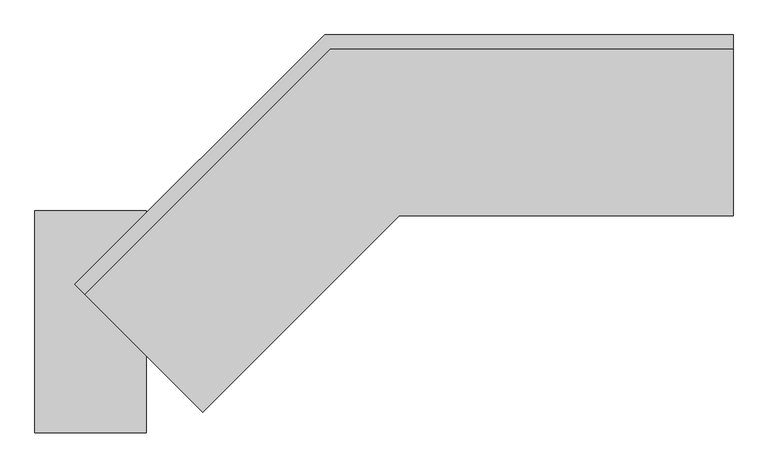
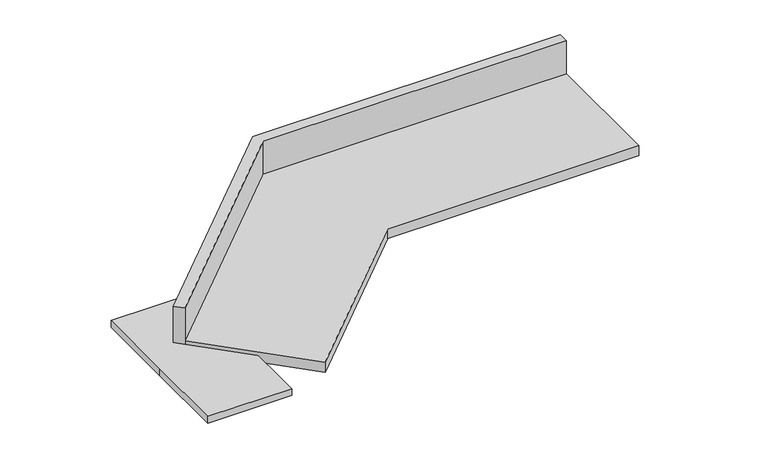
"""IFC4 building model written with IfcOpenShell, lengths in millimetres: proxy geometry, CT020 - Countertop, SS, No Opening - Angled, L-Shaped : CT020 - Countertop, SS, No Opening - Angled, L-Shaped."""

from ifc_helpers import new_model, si_unit, frame, origin, place, context, project, spatial, polyline, outline, extrude, source, transform, mapped, element, save


def specialty_equipment_98d5d29f(model_context):
    return source(origin(), model_context, "Body", "SweptSolid", [
        extrude(outline(polyline([(656.9660168, 747.8563381), (-15.7601301, 75.1301912), (-42.7008985, 102.0709596), (641.1844801, 785.9563381), (1760.7444575, 785.9563381), (1760.7444575, 747.8563381), (656.9660168, 747.8563381)])), frame((0.0, 0.0, 838.2), z_axis=(0.0, 0.0, 1.0), x_axis=(1.0, 0.0, 0.0)), (0.0, 0.0, 1.0), 165.1),
        extrude(outline(polyline([(1760.7444575, 290.6563381), (846.3444575, 290.6563381), (307.5290903, -248.1590292), (-15.7601301, 75.1301912), (656.9660168, 747.8563381), (1760.7444575, 747.8563381), (1760.7444575, 290.6563381)])), frame((0.0, 0.0, 838.2), z_axis=(0.0, 0.0, 1.0), x_axis=(1.0, 0.0, 0.0)), (0.0, 0.0, 1.0), 38.1),
        extrude(outline(polyline([(-152.4, 304.8), (152.4, 304.8), (152.4, -304.8), (-152.4, -304.8), (-152.4, 0.0), (-152.4, 304.8)])), frame((0.0, 0.0, 838.2), z_axis=(0.0, 0.0, 1.0), x_axis=(1.0, 0.0, 0.0)), (0.0, 0.0, 1.0), 25.4),
    ])


if __name__ == "__main__":
    model = new_model("IFC4")
    model_context = context("Model", 3, world=origin())
    ifc_project = project(units=[si_unit("LENGTHUNIT", "METRE", prefix="MILLI")], contexts=[model_context])
    site = spatial("IfcSite", under=ifc_project)
    building = spatial("IfcBuilding", under=site)
    placement = place(None, origin())
    specialty_equipment_shape = specialty_equipment_98d5d29f(model_context)
    element("IfcBuildingElementProxy", 1, Name="CT020 - Countertop, SS, No Opening - Angled, L-Shaped : CT020 - Countertop, SS, No Opening - Angled, L-Shaped", ObjectType="CT020 - Countertop, SS, No Opening - Angled, L-Shaped : CT020 - Countertop, SS, No Opening - Angled, L-Shaped", at=placement, inside=building, context=model_context, shape_type="MappedRepresentation", body=[
        mapped(specialty_equipment_shape, transform((0.0, 0.0, 0.0), x_axis=(1.0, 0.0, 0.0), y_axis=(0.0, 1.0, 0.0), z_axis=(0.0, 0.0, 1.0))),
    ])
    save(model, "model.ifc")

# Revit data of these elements
# Type "CT020 - Countertop, SS, No Opening - Angled, L-Shaped : CT020 - Countertop, SS, No Opening - Angled, L-Shaped"
#   Watts2 = "0"
#   Watts1 = "0"
#   Unit_Issue = "LF"
#   UTIL_6_Misc = "-"
#   UTIL_5_NonMedGas = "-"
#   UTIL_4_MiscGas = "-"
#   UTIL_3_MedGas = "-"
#   UTIL_2_Elec = "-"
#   UTIL_1_WaterDrain = "-"
#   Nomenclature = "Countertop, Solid Surface"
#   NSN = ""
#   Location [instance default] = ""
#   JSN = "CT020"
#   Fund_Source_VA = "-"
#   Fund_Source_Navy = "-"
#   Fund_Source_Army = "-"
#   Fund_Source_AF = "-"
#   ELEC_Volts2 = "0"
#   ELEC_Volts1 = "0"
#   ELEC_Phase2 = "0"
#   ELEC_Phase1 = "0"
#   ELEC_HertzSwitch = "0"
#   ELEC_HertzDependent = "0"
#   ELEC_Hertz = "0"
#   ELEC_Amps2 = "0"
#   ELEC_Amps1 = "0"
#   DetailDescription = ""
#   CAT_VA = "A"
#   CAT_Navy = "A"
#   CAT_IHS = "-"
#   CAT_Army = "A"
#   CAT_AF = "A"
#   BTUperhour = "0"
#   Weight_IP = 14
#   DIM_Width_IP = 1' - 0"
#   DIM_Height_IP = 0' - 1"
#   DIM_Depth_IP = 2' - 0"
#   CustomLength [instance default] = 4' - 0"
#   Assembly Code = ""
# Element 1 (IfcBuildingElementProxy, "CT020 - Countertop, SS, No Opening - Angled, L-Shaped : CT020 - Countertop, SS, No Opening - Angled, L-Shaped")
#   Materials on its faces: "CounterTopFinish", "EquipSpace"
# Materials
#   "CounterTopFinish": class "Unassigned", colour RGB 139 121 96, transparency 0
#   "EquipSpace": class "Unassigned", colour RGB 221 217 195, transparency 0.5
